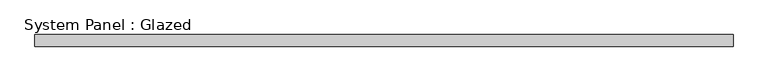
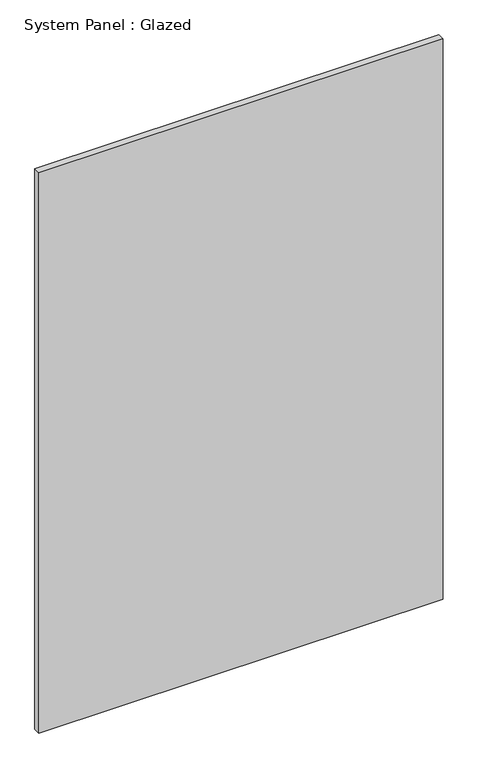
"""IFC4 building model written with IfcOpenShell, lengths in millimetres: plate geometry, System Panel : Glazed."""

import ifcopenshell
import ifcopenshell.guid

model = None  # the IFC model being written
_history = None  # IfcOwnerHistory: only IFC2X3 demands one
_inside = {}  # id of a spatial element -> (the spatial element, [elements in it])
_under = {}  # id of a project, library or spatial element -> (it, [spatial elements below it])
_declared = {}  # id of a project -> (the project, [libraries it declares])
_typed = {}  # id of a type object -> (the type object, [elements of that type])
_made_of = {}  # id of a material, layer set ... -> (it, [elements and type objects made of it])


def new_model(schema):
    """Start an empty IFC model of exactly this schema.

    Asked for "IFC4X3", IfcOpenShell would pick the latest addendum, in which some entities
    have other attributes; the version numbers below select the first issue.
    IFC2X3 requires an IfcOwnerHistory on every rooted entity: one is made here for all.
    """
    global model, _history
    if schema == "IFC4X3":
        model = ifcopenshell.file(schema_version=(4, 3, 0, 0))
    else:
        model = ifcopenshell.file(schema=schema)
    _inside.clear()
    _under.clear()
    _declared.clear()
    _typed.clear()
    _made_of.clear()
    _history = None
    if model.schema == "IFC2X3":
        org = make("IfcOrganization", Name="unknown")
        user = make(
            "IfcPersonAndOrganization",
            ThePerson=make("IfcPerson", FamilyName="unknown"),
            TheOrganization=org,
        )
        app = make(
            "IfcApplication",
            ApplicationDeveloper=org,
            Version="unknown",
            ApplicationFullName="unknown",
            ApplicationIdentifier="unknown",
        )
        _history = make(
            "IfcOwnerHistory",
            OwningUser=user,
            OwningApplication=app,
            ChangeAction="ADDED",
            CreationDate=0,
        )
    return model


def make(cls, **values):
    """One entity of the class cls with the attributes given. An attribute that is None is left unset."""
    return model.create_entity(
        cls, **{name: value for name, value in values.items() if value is not None}
    )


def rooted(cls, **values):
    """An entity with a GlobalId (a new one), such as an element, a storey or a relation."""
    return make(cls, GlobalId=ifcopenshell.guid.new(), OwnerHistory=_history, **values)


def si_unit(unit_type, name, prefix=None):
    """IfcSIUnit, for example si_unit("LENGTHUNIT", "METRE", prefix="MILLI")."""
    return make("IfcSIUnit", UnitType=unit_type, Prefix=prefix, Name=name)


def assignment(units):
    """IfcUnitAssignment: the units of a project."""
    return None if units is None else make("IfcUnitAssignment", Units=units)


def point(xyz):
    """IfcCartesianPoint."""
    return None if xyz is None else make("IfcCartesianPoint", Coordinates=xyz)


def direction(xyz):
    """IfcDirection."""
    return None if xyz is None else make("IfcDirection", DirectionRatios=xyz)


def frame(location, z_axis=None, x_axis=None):
    """IfcAxis2Placement3D, a coordinate frame: its origin and axes. An axis left out is left unset."""
    return make(
        "IfcAxis2Placement3D",
        Location=point(location),
        Axis=direction(z_axis),
        RefDirection=direction(x_axis),
    )


def origin():
    """The frame at (0, 0, 0) with its axes left unset."""
    return frame((0.0, 0.0, 0.0))


def origin_with_axes():
    """The frame at (0, 0, 0) with the z axis (0, 0, 1) and the x axis (1, 0, 0) written out."""
    return frame((0.0, 0.0, 0.0), z_axis=(0.0, 0.0, 1.0), x_axis=(1.0, 0.0, 0.0))


def place(relative_to, where):
    """IfcLocalPlacement: puts the frame where relative to a parent placement (None: the world)."""
    return make(
        "IfcLocalPlacement", PlacementRelTo=relative_to, RelativePlacement=where
    )


def context(
    kind, dimensions, precision=None, world=None, true_north=None, identifier=None
):
    """IfcGeometricRepresentationContext, for example the 3D "Model" context."""
    return make(
        "IfcGeometricRepresentationContext",
        ContextIdentifier=identifier,
        ContextType=kind,
        CoordinateSpaceDimension=dimensions,
        Precision=precision,
        WorldCoordinateSystem=world,
        TrueNorth=true_north,
    )


def project(units=None, contexts=None):
    """IfcProject with its units and contexts."""
    return rooted(
        "IfcProject",
        Name="project",
        RepresentationContexts=contexts,
        UnitsInContext=assignment(units),
    )


def spatial(cls, under=None, at=None, **own):
    """A site, building, storey or space (cls), placed at a placement, below another one or the project."""
    s = rooted(cls, ObjectPlacement=at, **own)
    if under is not None:
        _under.setdefault(under.id(), (under, []))[1].append(s)
    return s


def polyline(points):
    """IfcPolyline through the points."""
    return make("IfcPolyline", Points=[point(p) for p in points])


def outline(outer, holes=None, kind="AREA"):
    """IfcArbitraryClosedProfileDef: a profile drawn as a closed curve; with holes, ...WithVoids."""
    if holes is None:
        return make("IfcArbitraryClosedProfileDef", ProfileType=kind, OuterCurve=outer)
    return make(
        "IfcArbitraryProfileDefWithVoids",
        ProfileType=kind,
        OuterCurve=outer,
        InnerCurves=holes,
    )


def extrude(swept, where, along, depth):
    """IfcExtrudedAreaSolid: the profile swept, set in the frame where, extruded along a direction by depth."""
    return make(
        "IfcExtrudedAreaSolid",
        SweptArea=swept,
        Position=where,
        ExtrudedDirection=direction(along),
        Depth=depth,
    )


def shape(context_of_items, identifier, shape_type, items):
    """IfcShapeRepresentation: the items that make up one representation, for example the "Body"."""
    return make(
        "IfcShapeRepresentation",
        ContextOfItems=context_of_items,
        RepresentationIdentifier=identifier,
        RepresentationType=shape_type,
        Items=items,
    )


def source(mapping_origin, context_of_items, identifier, shape_type, items):
    """IfcRepresentationMap: a shape defined once, which mapped items show again and again."""
    return make(
        "IfcRepresentationMap",
        MappingOrigin=mapping_origin,
        MappedRepresentation=shape(context_of_items, identifier, shape_type, items),
    )


def transform(
    local_origin,
    x_axis=None,
    y_axis=None,
    z_axis=None,
    scale=None,
    scale2=None,
    scale3=None,
    uniform=True,
):
    """IfcCartesianTransformationOperator3D, or its non-uniform kind. x_axis, y_axis, z_axis: its Axis1, 2, 3."""
    if uniform:
        return make(
            "IfcCartesianTransformationOperator3D",
            Axis1=direction(x_axis),
            Axis2=direction(y_axis),
            LocalOrigin=point(local_origin),
            Scale=scale,
            Axis3=direction(z_axis),
        )
    return make(
        "IfcCartesianTransformationOperator3DnonUniform",
        Axis1=direction(x_axis),
        Axis2=direction(y_axis),
        LocalOrigin=point(local_origin),
        Scale=scale,
        Axis3=direction(z_axis),
        Scale2=scale2,
        Scale3=scale3,
    )


def mapped(mapping_source, mapping_target):
    """IfcMappedItem: shows the shape of a source again, moved by a transform."""
    return make(
        "IfcMappedItem", MappingSource=mapping_source, MappingTarget=mapping_target
    )


def made_of(thing, what):
    """Note that an element or type object is made of a material, layer set ...; save() writes the relation."""
    if what is not None:
        _made_of.setdefault(what.id(), (what, []))[1].append(thing)
    return thing


def element(
    cls,
    number,
    at=None,
    inside=None,
    cuts=None,
    type_object=None,
    material=None,
    context=None,
    identifier="Body",
    shape_type=None,
    held_by="IfcProductDefinitionShape",
    body=None,
    shapes=None,
    **own,
):
    """One element of the class cls, such as IfcWall. Its Tag is "e" and its number.

    at: its placement. inside: the storey or other place that contains it. cuts: it is an
    opening in that element (IfcRelVoidsElement). A single representation is given by context,
    identifier, shape_type and body (its items); several are given by shapes. held_by: the class
    of the entity that holds the representations. save() writes the other relations.
    """
    e = rooted(cls, Tag="e%d" % number, ObjectPlacement=at, **own)
    if body is not None:
        shapes = [shape(context, identifier, shape_type, body)]
    if shapes is not None:
        e.Representation = make(held_by, Representations=shapes)
    if inside is not None:
        _inside.setdefault(inside.id(), (inside, []))[1].append(e)
    if cuts is not None:
        rooted(
            "IfcRelVoidsElement", RelatingBuildingElement=cuts, RelatedOpeningElement=e
        )
    if type_object is not None:
        _typed.setdefault(type_object.id(), (type_object, []))[1].append(e)
    return made_of(e, material)


def aggregate(whole, parts):
    """IfcRelAggregates: a whole, such as a stair, and the parts it consists of."""
    return rooted("IfcRelAggregates", RelatingObject=whole, RelatedObjects=parts)


def save(model, path):
    """Write the relations noted so far, then the file.

    IfcRelAggregates (storeys below a building ...), IfcRelContainedInSpatialStructure (elements
    in a storey), IfcRelDefinesByType, IfcRelAssociatesMaterial and IfcRelDeclares: one each for
    every whole, place, type object, material and project.
    """
    for whole, parts in _under.values():
        aggregate(whole, parts)
    for where, things in _inside.values():
        rooted(
            "IfcRelContainedInSpatialStructure",
            RelatedElements=things,
            RelatingStructure=where,
        )
    for kind, things in _typed.values():
        rooted("IfcRelDefinesByType", RelatedObjects=things, RelatingType=kind)
    for what, things in _made_of.values():
        rooted("IfcRelAssociatesMaterial", RelatedObjects=things, RelatingMaterial=what)
    for by, libraries in _declared.values():
        rooted("IfcRelDeclares", RelatingContext=by, RelatedDefinitions=libraries)
    model.write(path)


def system_panel_glazed_c51f38ac(model_context):
    return source(origin(), model_context, "Body", "SweptSolid", [
        extrude(outline(polyline([(725.0514967, -49.5), (-725.0514967, -49.5), (-725.0514967, -24.5), (725.0514967, -24.5), (725.0514967, -49.5)])), origin_with_axes(), (0.0, 0.0, 1.0), 2125.0),
    ])


if __name__ == "__main__":
    model = new_model("IFC4")
    model_context = context("Model", 3, world=origin())
    ifc_project = project(units=[si_unit("LENGTHUNIT", "METRE", prefix="MILLI")], contexts=[model_context])
    site = spatial("IfcSite", under=ifc_project)
    building = spatial("IfcBuilding", under=site)
    placement = place(None, origin())
    system_panel_glazed_shape = system_panel_glazed_c51f38ac(model_context)
    element("IfcPlate", 1, ObjectType="System Panel : Glazed", at=placement, inside=building, context=model_context, shape_type="MappedRepresentation", body=[
        mapped(system_panel_glazed_shape, transform((0.0, 0.0, 0.0), x_axis=(1.0, 0.0, 0.0), y_axis=(0.0, 1.0, 0.0), z_axis=(0.0, 0.0, 1.0))),
    ])
    save(model, "model.ifc")

# Revit data of these elements
# Type "System Panel : Glazed"
#   Keynote = "H11"
#   Construction Type Id = "GSP4R"
#   Analytic Construction = "1/8 in Pilkington single glazing"
#   Visual Light Transmittance = 0.9
#   Solar Heat Gain Coefficient = 0.86
#   Heat Transfer Coefficient (U) = 6.7069 W/(m²·K)
# Element 1 (IfcPlate, "System Panel : Glazed")
#   Materials on its faces: "Glass"
# Materials
#   "Glass": class "Glass", colour RGB 0 128 192, transparency 0.9, Description = "Soda Lime Glass", Cost = 0
